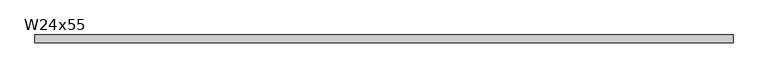
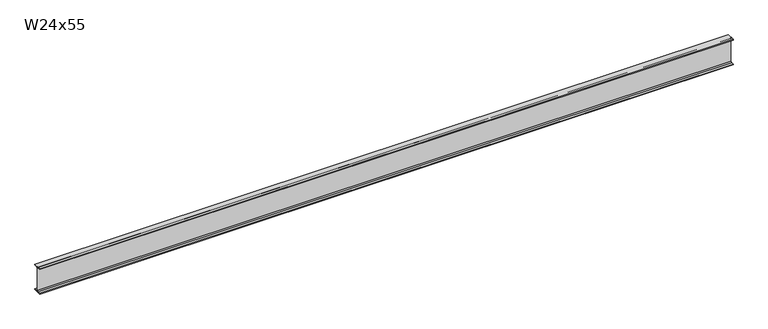
"""IFC4 building model written with IfcOpenShell, lengths in millimetres: beam geometry, RME W-Wide Flange : W24x55."""

import ifcopenshell
import ifcopenshell.guid

model = None  # the IFC model being written
_history = None  # IfcOwnerHistory: only IFC2X3 demands one
_inside = {}  # id of a spatial element -> (the spatial element, [elements in it])
_under = {}  # id of a project, library or spatial element -> (it, [spatial elements below it])
_declared = {}  # id of a project -> (the project, [libraries it declares])
_typed = {}  # id of a type object -> (the type object, [elements of that type])
_made_of = {}  # id of a material, layer set ... -> (it, [elements and type objects made of it])


def new_model(schema):
    """Start an empty IFC model of exactly this schema.

    Asked for "IFC4X3", IfcOpenShell would pick the latest addendum, in which some entities
    have other attributes; the version numbers below select the first issue.
    IFC2X3 requires an IfcOwnerHistory on every rooted entity: one is made here for all.
    """
    global model, _history
    if schema == "IFC4X3":
        model = ifcopenshell.file(schema_version=(4, 3, 0, 0))
    else:
        model = ifcopenshell.file(schema=schema)
    _inside.clear()
    _under.clear()
    _declared.clear()
    _typed.clear()
    _made_of.clear()
    _history = None
    if model.schema == "IFC2X3":
        org = make("IfcOrganization", Name="unknown")
        user = make(
            "IfcPersonAndOrganization",
            ThePerson=make("IfcPerson", FamilyName="unknown"),
            TheOrganization=org,
        )
        app = make(
            "IfcApplication",
            ApplicationDeveloper=org,
            Version="unknown",
            ApplicationFullName="unknown",
            ApplicationIdentifier="unknown",
        )
        _history = make(
            "IfcOwnerHistory",
            OwningUser=user,
            OwningApplication=app,
            ChangeAction="ADDED",
            CreationDate=0,
        )
    return model


def make(cls, **values):
    """One entity of the class cls with the attributes given. An attribute that is None is left unset."""
    return model.create_entity(
        cls, **{name: value for name, value in values.items() if value is not None}
    )


def rooted(cls, **values):
    """An entity with a GlobalId (a new one), such as an element, a storey or a relation."""
    return make(cls, GlobalId=ifcopenshell.guid.new(), OwnerHistory=_history, **values)


def si_unit(unit_type, name, prefix=None):
    """IfcSIUnit, for example si_unit("LENGTHUNIT", "METRE", prefix="MILLI")."""
    return make("IfcSIUnit", UnitType=unit_type, Prefix=prefix, Name=name)


def assignment(units):
    """IfcUnitAssignment: the units of a project."""
    return None if units is None else make("IfcUnitAssignment", Units=units)


def point(xyz):
    """IfcCartesianPoint."""
    return None if xyz is None else make("IfcCartesianPoint", Coordinates=xyz)


def direction(xyz):
    """IfcDirection."""
    return None if xyz is None else make("IfcDirection", DirectionRatios=xyz)


def frame(location, z_axis=None, x_axis=None):
    """IfcAxis2Placement3D, a coordinate frame: its origin and axes. An axis left out is left unset."""
    return make(
        "IfcAxis2Placement3D",
        Location=point(location),
        Axis=direction(z_axis),
        RefDirection=direction(x_axis),
    )


def frame_2d(location, x_axis=None):
    """IfcAxis2Placement2D, a coordinate frame in the plane: its origin and x axis."""
    return make(
        "IfcAxis2Placement2D", Location=point(location), RefDirection=direction(x_axis)
    )


def origin():
    """The frame at (0, 0, 0) with its axes left unset."""
    return frame((0.0, 0.0, 0.0))


def place(relative_to, where):
    """IfcLocalPlacement: puts the frame where relative to a parent placement (None: the world)."""
    return make(
        "IfcLocalPlacement", PlacementRelTo=relative_to, RelativePlacement=where
    )


def context(
    kind, dimensions, precision=None, world=None, true_north=None, identifier=None
):
    """IfcGeometricRepresentationContext, for example the 3D "Model" context."""
    return make(
        "IfcGeometricRepresentationContext",
        ContextIdentifier=identifier,
        ContextType=kind,
        CoordinateSpaceDimension=dimensions,
        Precision=precision,
        WorldCoordinateSystem=world,
        TrueNorth=true_north,
    )


def project(units=None, contexts=None):
    """IfcProject with its units and contexts."""
    return rooted(
        "IfcProject",
        Name="project",
        RepresentationContexts=contexts,
        UnitsInContext=assignment(units),
    )


def spatial(cls, under=None, at=None, **own):
    """A site, building, storey or space (cls), placed at a placement, below another one or the project."""
    s = rooted(cls, ObjectPlacement=at, **own)
    if under is not None:
        _under.setdefault(under.id(), (under, []))[1].append(s)
    return s


def polyline(points):
    """IfcPolyline through the points."""
    return make("IfcPolyline", Points=[point(p) for p in points])


def circle_curve(where, radius):
    """IfcCircle in the frame where."""
    return make("IfcCircle", Position=where, Radius=radius)


def trimmed(basis, trim1, trim2, sense, master):
    """IfcTrimmedCurve: the piece of a basis curve between two trims."""
    return make(
        "IfcTrimmedCurve",
        BasisCurve=basis,
        Trim1=trim1,
        Trim2=trim2,
        SenseAgreement=sense,
        MasterRepresentation=master,
    )


def segment(curve, same_sense, transition):
    """IfcCompositeCurveSegment."""
    return make(
        "IfcCompositeCurveSegment",
        Transition=transition,
        SameSense=same_sense,
        ParentCurve=curve,
    )


def composite_curve(segments, self_intersect=None):
    """IfcCompositeCurve: segments joined end to end."""
    return make("IfcCompositeCurve", Segments=segments, SelfIntersect=self_intersect)


def outline(outer, holes=None, kind="AREA"):
    """IfcArbitraryClosedProfileDef: a profile drawn as a closed curve; with holes, ...WithVoids."""
    if holes is None:
        return make("IfcArbitraryClosedProfileDef", ProfileType=kind, OuterCurve=outer)
    return make(
        "IfcArbitraryProfileDefWithVoids",
        ProfileType=kind,
        OuterCurve=outer,
        InnerCurves=holes,
    )


def extrude(swept, where, along, depth):
    """IfcExtrudedAreaSolid: the profile swept, set in the frame where, extruded along a direction by depth."""
    return make(
        "IfcExtrudedAreaSolid",
        SweptArea=swept,
        Position=where,
        ExtrudedDirection=direction(along),
        Depth=depth,
    )


def shape(context_of_items, identifier, shape_type, items):
    """IfcShapeRepresentation: the items that make up one representation, for example the "Body"."""
    return make(
        "IfcShapeRepresentation",
        ContextOfItems=context_of_items,
        RepresentationIdentifier=identifier,
        RepresentationType=shape_type,
        Items=items,
    )


def source(mapping_origin, context_of_items, identifier, shape_type, items):
    """IfcRepresentationMap: a shape defined once, which mapped items show again and again."""
    return make(
        "IfcRepresentationMap",
        MappingOrigin=mapping_origin,
        MappedRepresentation=shape(context_of_items, identifier, shape_type, items),
    )


def transform(
    local_origin,
    x_axis=None,
    y_axis=None,
    z_axis=None,
    scale=None,
    scale2=None,
    scale3=None,
    uniform=True,
):
    """IfcCartesianTransformationOperator3D, or its non-uniform kind. x_axis, y_axis, z_axis: its Axis1, 2, 3."""
    if uniform:
        return make(
            "IfcCartesianTransformationOperator3D",
            Axis1=direction(x_axis),
            Axis2=direction(y_axis),
            LocalOrigin=point(local_origin),
            Scale=scale,
            Axis3=direction(z_axis),
        )
    return make(
        "IfcCartesianTransformationOperator3DnonUniform",
        Axis1=direction(x_axis),
        Axis2=direction(y_axis),
        LocalOrigin=point(local_origin),
        Scale=scale,
        Axis3=direction(z_axis),
        Scale2=scale2,
        Scale3=scale3,
    )


def mapped(mapping_source, mapping_target):
    """IfcMappedItem: shows the shape of a source again, moved by a transform."""
    return make(
        "IfcMappedItem", MappingSource=mapping_source, MappingTarget=mapping_target
    )


def made_of(thing, what):
    """Note that an element or type object is made of a material, layer set ...; save() writes the relation."""
    if what is not None:
        _made_of.setdefault(what.id(), (what, []))[1].append(thing)
    return thing


def element(
    cls,
    number,
    at=None,
    inside=None,
    cuts=None,
    type_object=None,
    material=None,
    context=None,
    identifier="Body",
    shape_type=None,
    held_by="IfcProductDefinitionShape",
    body=None,
    shapes=None,
    **own,
):
    """One element of the class cls, such as IfcWall. Its Tag is "e" and its number.

    at: its placement. inside: the storey or other place that contains it. cuts: it is an
    opening in that element (IfcRelVoidsElement). A single representation is given by context,
    identifier, shape_type and body (its items); several are given by shapes. held_by: the class
    of the entity that holds the representations. save() writes the other relations.
    """
    e = rooted(cls, Tag="e%d" % number, ObjectPlacement=at, **own)
    if body is not None:
        shapes = [shape(context, identifier, shape_type, body)]
    if shapes is not None:
        e.Representation = make(held_by, Representations=shapes)
    if inside is not None:
        _inside.setdefault(inside.id(), (inside, []))[1].append(e)
    if cuts is not None:
        rooted(
            "IfcRelVoidsElement", RelatingBuildingElement=cuts, RelatedOpeningElement=e
        )
    if type_object is not None:
        _typed.setdefault(type_object.id(), (type_object, []))[1].append(e)
    return made_of(e, material)


def aggregate(whole, parts):
    """IfcRelAggregates: a whole, such as a stair, and the parts it consists of."""
    return rooted("IfcRelAggregates", RelatingObject=whole, RelatedObjects=parts)


def save(model, path):
    """Write the relations noted so far, then the file.

    IfcRelAggregates (storeys below a building ...), IfcRelContainedInSpatialStructure (elements
    in a storey), IfcRelDefinesByType, IfcRelAssociatesMaterial and IfcRelDeclares: one each for
    every whole, place, type object, material and project.
    """
    for whole, parts in _under.values():
        aggregate(whole, parts)
    for where, things in _inside.values():
        rooted(
            "IfcRelContainedInSpatialStructure",
            RelatedElements=things,
            RelatingStructure=where,
        )
    for kind, things in _typed.values():
        rooted("IfcRelDefinesByType", RelatedObjects=things, RelatingType=kind)
    for what, things in _made_of.values():
        rooted("IfcRelAssociatesMaterial", RelatedObjects=things, RelatingMaterial=what)
    for by, libraries in _declared.values():
        rooted("IfcRelDeclares", RelatingContext=by, RelatedDefinitions=libraries)
    model.write(path)


def w24x55_3b0f53b1(model_context):
    return source(origin(), model_context, "Body", "SweptSolid", [
        extrude(outline(composite_curve([segment(polyline([(89.027, -286.893), (89.027, -299.72), (-89.027, -299.72), (-89.027, -286.893), (-28.702, -286.893)]), True, "CONTINUOUS"), segment(trimmed(circle_curve(frame_2d((-28.702, -263.2075)), 23.6855), [point((-28.702, -286.893))], [point((-5.0165, -263.2075))], True, "CARTESIAN"), True, "CONTINUOUS"), segment(polyline([(-5.0165, -263.2075), (-5.0165, 263.2075)]), True, "CONTINUOUS"), segment(trimmed(circle_curve(frame_2d((-28.702, 263.2075)), 23.6855), [point((-5.0165, 263.2075))], [point((-28.702, 286.893))], True, "CARTESIAN"), True, "CONTINUOUS"), segment(polyline([(-28.702, 286.893), (-89.027, 286.893), (-89.027, 299.72), (89.027, 299.72), (89.027, 286.893), (28.702, 286.893)]), True, "CONTINUOUS"), segment(trimmed(circle_curve(frame_2d((28.702, 263.2075)), 23.6855), [point((28.702, 286.893))], [point((5.0165, 263.2075))], True, "CARTESIAN"), True, "CONTINUOUS"), segment(polyline([(5.0165, 263.2075), (5.0165, -263.2075)]), True, "CONTINUOUS"), segment(trimmed(circle_curve(frame_2d((28.702, -263.2075)), 23.6855), [point((5.0165, -263.2075))], [point((28.702, -286.893))], True, "CARTESIAN"), True, "CONTINUOUS"), segment(polyline([(28.702, -286.893), (89.027, -286.893)]), True, "CONTINUOUS")], self_intersect=False)), frame((-7750.213533, 0.0, 0.0), z_axis=(1.0, 0.0, 0.0), x_axis=(0.0, 1.0, 0.0)), (0.0, 0.0, 1.0), 15500.4270661),
    ])


if __name__ == "__main__":
    model = new_model("IFC4")
    model_context = context("Model", 3, world=origin())
    ifc_project = project(units=[si_unit("LENGTHUNIT", "METRE", prefix="MILLI")], contexts=[model_context])
    site = spatial("IfcSite", under=ifc_project)
    building = spatial("IfcBuilding", under=site)
    placement = place(None, origin())
    w24x55_shape = w24x55_3b0f53b1(model_context)
    element("IfcBeam", 1, ObjectType="RME W-Wide Flange : W24x55", at=placement, inside=building, context=model_context, shape_type="MappedRepresentation", body=[
        mapped(w24x55_shape, transform((0.0, 0.0, 0.0), x_axis=(1.0, 0.0, 0.0), y_axis=(0.0, 1.0, 0.0), z_axis=(0.0, 0.0, 1.0))),
    ])
    save(model, "model.ifc")

# Revit data of these elements
# Type "RME W-Wide Flange : W24x55"
#   WELD P [instance default] = ""
#   WELD LE [instance default] = ""
#   WELD D [instance default] = ""
#   TOP SECTION SIZE [instance default] = ""
#   TOP SECTION LENGTH [instance default] = ""
#   REMARKS [instance default] = ""
#   REINF TYPE [instance default] = ""
#   Nominal Size = "W24"
#   End Bearing Capacity [instance default] = ""
#   BOT SECTION SIZE [instance default] = ""
#   BOT SECTION LENGTH [instance default] = ""
#   Assembly Code = "B10"
#   W = 55
#   Start Extension Calculation [instance default] = 10' - 0"
#   Start Extension [instance default] = -0' - 0 1/2"
#   End Extension Calculation [instance default] = 10' - 0"
#   End Extension [instance default] = -0' - 0 1/2"
#   Length [instance default] = 5' - 0"
#   bf = 0' - 7.01"
#   d = 1' - 11.6"
#   k = 0' - 1 7/16"
#   k2 = 0' - 0.9325"
#   tf = 0' - 0.505"
#   tw = 0' - 0.395"
#   A = 0.1125 SF
#   Structural Material [instance default] = Metal - Steel - ASTM A992
# Element 1 (IfcBeam, "RME W-Wide Flange : W24x55")
#   Length = 50' - 10.25303"
#   Materials on its faces: "Metal - Steel - ASTM A992"
# Materials
#   "Metal - Steel - ASTM A992": class "Metal", colour RGB 255 128 0, transparency 0
